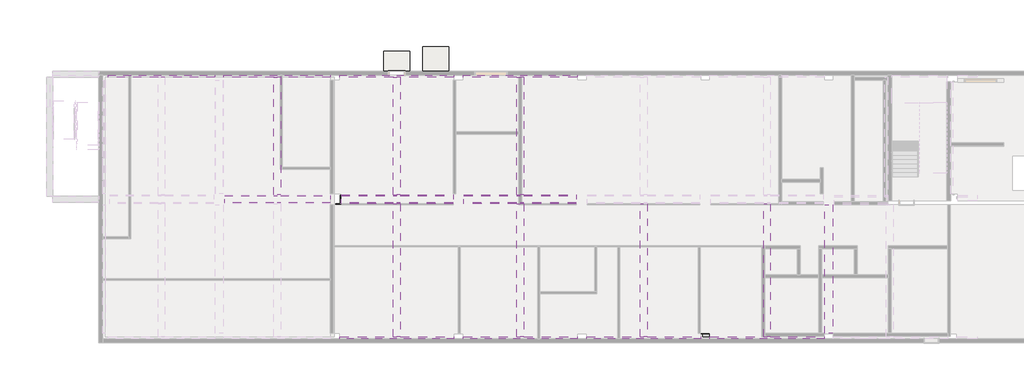
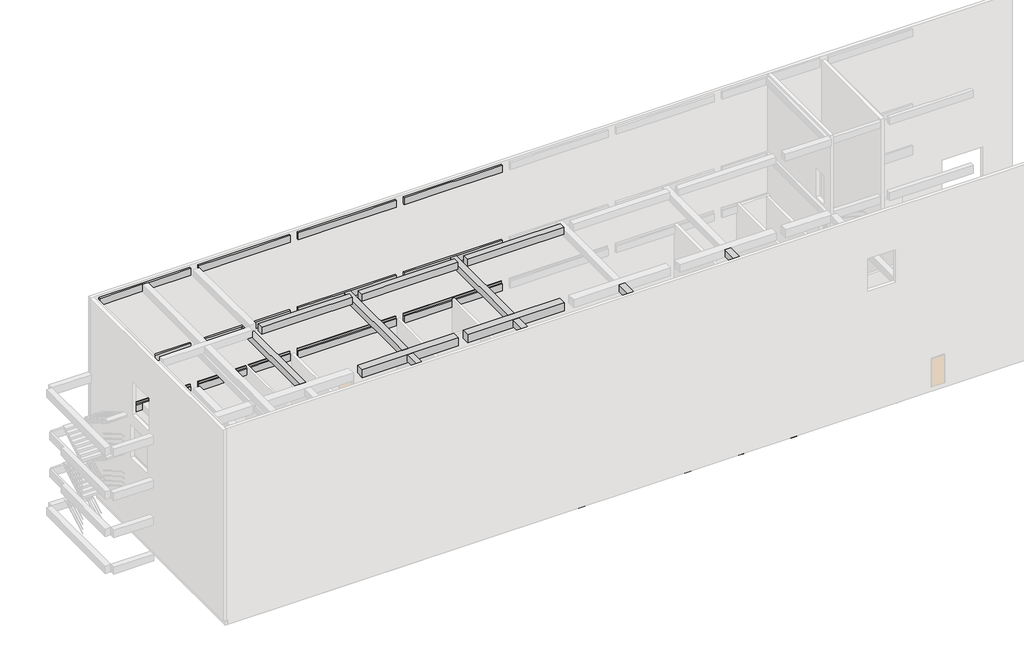
# One storey, part 3 of 5: 54 beams, 2 slabs.
# Revit data of these elements (continued)
# Room at (45344.344, 10064.78) mm, phase "New Construction", upper level "TOC", upper offset 3000 mm, lower offset 0 mm (continued)
#   H_Wall-Base Material-3 = ""
#   H_Floor-Base Material-1 = "Concrete Slab"
#   H_Floor-Base Material-2 = "Steel Trowel Finish"
#   H_Floor-Base Material-3 = ""
#   H_Floor-Base Material-4 = "Concrete Slab"
#   H_Floor-Base Material-5 = ""
#   H_Floor Finish-1 = "Screed"
#   H_Floor Finish-2 = ""
#   H_Floor Finish Remark = "Vinyl Tile"
#   H_Skirt Base Material = "Same as Wall"
#   H_Skirt-Base Material-1 = ""
#   H_Skirt-Base Material-2 = ""
#   H_Skirt-Base Material-3 = ""
#   H_Skirt-Base Material-4 = ""
#   H_Skirt-Base Material-5 = ""
#   H_Skirt Finish-1 = "Vinyl Tile"
#   H_Skirt Finish-2 = ""
#   H_Wall Finish Style Name = "Water Emulsion Paint"
#   H_Wall Base Material = "Masonry Wall / Cement Plaster"
#   H_Wall-Base Material-4 = ""
#   H_Wall-Base Material-5 = ""
#   H_Wall Finish-1 = "Water Emulsion Paint"
#   H_Wall Finish-2 = ""
#   H_Ceiling Finish Style Name = "Suspended Gypsum Plaster Board Ceiling (M-Bar)"
#   H_Ceiling Base Material = "Concrete Slab / Fair Faced Concrete"
#   H_Ceiling-Base Material-1 = "(Concrete Slab)"
#   H_Ceiling-Base Material-2 = "(Fair Faced Concrete)"
#   H_Ceiling-Base Material-3 = ""
#   H_Ceiling-Base Material-4 = ""
#   H_Ceiling-Base Material-5 = "Gypsum Plaster Board Ceiling System"
#   H_Ceiling Finish-1 = "Gypsum Plaster Board Ceiling System"
#   H_Ceiling Finish-2 = ""
#   H_Room W = 4700 mm
#   H_Room L = 8400 mm
#   H_Room H or CH = 3000 mm
#   Floor Finish Style No = F34B
#   Skirt Finish Style No = B35
#   Wall Finish Style No = W02A
#   Ceiling Finish Style No = C92
# Room at (49621.297, 12708.408) mm, phase "New Construction", upper level "TOC", upper offset 2700 mm, lower offset 0 mm
#   Comments = ""
#   Number = "109"
#   Name = "SHOWER ROOM"
#   H_Floor Finish Style Name = "Non-Slip Unglazed Ceramic Tile"
#   H_Floor Base Material = "Concrete Slab / Screed / Liquid Waterproof Membrane"
#   H_Wall-Base Material-1 = "Masonry Wall"
#   H_Skirt Finish Style Name = "Coved Vinyl Tile"
#   H_Wall-Base Material-2 = ""
#   H_Wall-Base Material-3 = ""
#   H_Floor-Base Material-1 = "Concrete Slab"
#   H_Floor-Base Material-2 = ""
#   H_Floor-Base Material-3 = "Screed"
#   H_Floor-Base Material-4 = "Concrete Slab"
#   H_Floor-Base Material-5 = ""
#   H_Floor Finish-1 = "Screed"
#   H_Floor Finish-2 = "Waterproof Membrane"
#   H_Floor Finish Remark = "Ceramic Tile"
#   H_Skirt Base Material = "Same as Wall"
#   H_Skirt-Base Material-1 = ""
#   H_Skirt-Base Material-2 = ""
#   H_Skirt-Base Material-3 = ""
#   H_Skirt-Base Material-4 = ""
#   H_Skirt-Base Material-5 = ""
#   H_Skirt Finish-1 = "Vinyl Tile"
#   H_Skirt Finish-2 = ""
#   H_Wall Finish Style Name = "Glazed Ceramic Tile (≤C.H+100) / No Paint (>C.H+100)"
#   H_Wall Base Material = "Masonry Wall / Waterproof Membrane"
#   H_Wall-Base Material-4 = "Waterproof Membrane"
#   H_Wall-Base Material-5 = "Glazed Ceramic Tile"
#   H_Wall Finish-1 = "Glazed Ceramic Tile"
#   H_Wall Finish-2 = ""
#   H_Ceiling Finish Style Name = "Suspended Acoustic Tiled Ceiling (M-Bar)"
#   H_Ceiling Base Material = "Concrete Slab / Fair Faced Concrete"
#   H_Ceiling-Base Material-1 = "(Concrete Slab)"
#   H_Ceiling-Base Material-2 = "(Fair Faced Concrete)"
#   H_Ceiling-Base Material-3 = ""
#   H_Ceiling-Base Material-4 = ""
#   H_Ceiling-Base Material-5 = "Acoustic Tiled Ceiling System (M-Bar)"
#   H_Ceiling Finish-1 = "Acoustic Tiled Ceiling System (M-Bar)"
#   H_Ceiling Finish-2 = ""
#   H_Room W = 2700 mm
#   H_Room L = 1400 mm
#   H_Room H or CH = 2700 mm
#   Floor Finish Style No = F31C
#   Skirt Finish Style No = none
#   Wall Finish Style No = W32F
#   Ceiling Finish Style No = C95A
# Room at (52871.108, 13591.136) mm, phase "New Construction", upper level "TOC", upper offset 5800 mm, lower offset 0 mm
#   Comments = ""
#   Number = "110"
#   Name = "STAIRCASE"
#   H_Floor Finish Style Name = "Vinyl Tile"
#   H_Floor Base Material = "Concrete Slab / Steel Trowel Finish"
#   H_Wall-Base Material-1 = "Concrete Wall"
#   H_Skirt Finish Style Name = "Coved Vinyl Tile"
#   H_Wall-Base Material-2 = "(Fair Faced Concrete)"
#   H_Wall-Base Material-3 = ""
#   H_Floor-Base Material-1 = "Concrete Slab"
#   H_Floor-Base Material-2 = "Steel Trowel Finish"
#   H_Floor-Base Material-3 = ""
#   H_Floor-Base Material-4 = "Concrete Slab"
#   H_Floor-Base Material-5 = "Steel Trowel Finish"
#   H_Floor Finish-1 = ""
#   H_Floor Finish-2 = ""
#   H_Floor Finish Remark = "Vinyl Tile"
#   H_Skirt Base Material = "Same as Wall"
#   H_Skirt-Base Material-1 = ""
#   H_Skirt-Base Material-2 = ""
#   H_Skirt-Base Material-3 = ""
#   H_Skirt-Base Material-4 = ""
#   H_Skirt-Base Material-5 = ""
#   H_Skirt Finish-1 = "Vinyl Tile"
#   H_Skirt Finish-2 = ""
#   H_Wall Finish Style Name = "Acrylic Emulsion Paint"
#   H_Wall Base Material = "Concrete Wall / Fair Faced Concrete"
#   H_Wall-Base Material-4 = ""
#   H_Wall-Base Material-5 = ""
#   H_Wall Finish-1 = "Acrylic Emulsion Paint"
#   H_Wall Finish-2 = ""
#   H_Ceiling Finish Style Name = "Acrylic Emulsion Paint"
#   H_Ceiling Base Material = "Concrete Slab / Fair Faced Concrete"
#   H_Ceiling-Base Material-1 = "(Concrete Slab)"
#   H_Ceiling-Base Material-2 = ""
#   H_Ceiling-Base Material-3 = ""
#   H_Ceiling-Base Material-4 = ""
#   H_Ceiling-Base Material-5 = ""
#   H_Ceiling Finish-1 = "Acrylic Emulsion Paint"
#   H_Ceiling Finish-2 = ""
#   H_Room W = 2000 mm
#   H_Room L = 8000 mm
#   H_Room H or CH = 5800 mm
#   Floor Finish Style No = F34A
#   Skirt Finish Style No = B35
#   Wall Finish Style No = W01A
#   Ceiling Finish Style No = C01
# Room at (56962.839, 14779.531) mm, phase "New Construction", upper level "TOC", upper offset 5800 mm, lower offset 0 mm
#   Comments = ""
#   Number = "124"
#   Name = "F.O TANK ROOM"
#   H_Floor Finish Style Name = "Non-Slip Epoxy Paint"
#   H_Floor Base Material = "Concrete Slab / Steel Trowel Finish"
#   H_Wall-Base Material-1 = "Concrete Wall"
#   H_Skirt Finish Style Name = "Epoxy Paint"
#   H_Wall-Base Material-2 = "(Fair Faced Concrete)"
#   H_Wall-Base Material-3 = ""
#   H_Floor-Base Material-1 = "Concrete Slab"
#   H_Floor-Base Material-2 = "Steel Trowel Finish"
#   H_Floor-Base Material-3 = ""
#   H_Floor-Base Material-4 = "Concrete Slab"
#   H_Floor-Base Material-5 = "Steel Trowel Finish"
#   H_Floor Finish-1 = ""
#   H_Floor Finish-2 = ""
#   H_Floor Finish Remark = ""
#   H_Skirt Base Material = "Same as Wall"
#   H_Skirt-Base Material-1 = ""
#   H_Skirt-Base Material-2 = ""
#   H_Skirt-Base Material-3 = ""
#   H_Skirt-Base Material-4 = ""
#   H_Skirt-Base Material-5 = ""
#   H_Skirt Finish-1 = "Epoxy Paint"
#   H_Skirt Finish-2 = ""
#   H_Wall Finish Style Name = "Acrylic Emulsion Paint"
#   H_Wall Base Material = "Masonry Wall / Cement Plaster"
#   H_Wall-Base Material-4 = ""
#   H_Wall-Base Material-5 = ""
#   H_Wall Finish-1 = "Acrylic Emulsion Paint"
#   H_Wall Finish-2 = ""
#   H_Ceiling Finish Style Name = "Acrylic Emulsion Paint"
#   H_Ceiling Base Material = "Concrete Slab / Fair Faced Concrete"
#   H_Ceiling-Base Material-1 = "(Concrete Slab)"
#   H_Ceiling-Base Material-2 = ""
#   H_Ceiling-Base Material-3 = ""
#   H_Ceiling-Base Material-4 = ""
#   H_Ceiling-Base Material-5 = ""
#   H_Ceiling Finish-1 = "Acrylic Emulsion Paint"
#   H_Ceiling Finish-2 = ""
#   H_Room W = 3800 mm
#   H_Room L = 8400 mm
#   H_Room H or CH = 5800 mm
#   Floor Finish Style No = F06A
#   Skirt Finish Style No = B03
#   Wall Finish Style No = W01A
#   Ceiling Finish Style No = C01
# Room at (61954.58, 4867.401) mm, phase "New Construction", upper level "TOC", upper offset 5800 mm, lower offset 0 mm
#   Comments = ""
#   Number = "125"
#   Name = "HVAC ROOM"
#   H_Floor Finish Style Name = "Non-Slip Epoxy Paint"
#   H_Floor Base Material = "Concrete Slab / Steel Trowel Finish"
#   H_Wall-Base Material-1 = "Concrete Wall"
#   H_Skirt Finish Style Name = "Epoxy Paint"
#   H_Wall-Base Material-2 = "(Fair Faced Concrete)"
#   H_Wall-Base Material-3 = ""
#   H_Floor-Base Material-1 = "Concrete Slab"
#   H_Floor-Base Material-2 = "Steel Trowel Finish"
#   H_Floor-Base Material-3 = ""
#   H_Floor-Base Material-4 = "Concrete Slab"
#   H_Floor-Base Material-5 = "Steel Trowel Finish"
#   H_Floor Finish-1 = ""
#   H_Floor Finish-2 = ""
#   H_Floor Finish Remark = ""
#   H_Skirt Base Material = "Same as Wall"
#   H_Skirt-Base Material-1 = ""
#   H_Skirt-Base Material-2 = ""
#   H_Skirt-Base Material-3 = ""
#   H_Skirt-Base Material-4 = ""
#   H_Skirt-Base Material-5 = ""
#   H_Skirt Finish-1 = "Epoxy Paint"
#   H_Skirt Finish-2 = ""
#   H_Wall Finish Style Name = "Acrylic Emulsion Paint"
#   H_Wall Base Material = "Masonry Wall / Cement Plaster"
#   H_Wall-Base Material-4 = ""
#   H_Wall-Base Material-5 = ""
#   H_Wall Finish-1 = "Acrylic Emulsion Paint"
#   H_Wall Finish-2 = ""
#   H_Ceiling Finish Style Name = "Suspended Acoustic Tiled Ceiling (M-Bar)"
#   H_Ceiling-Base Material-1 = "(Concrete Slab)"
#   H_Ceiling-Base Material-2 = "(Fair Faced Concrete)"
#   H_Ceiling-Base Material-3 = ""
#   H_Ceiling-Base Material-4 = ""
#   H_Ceiling-Base Material-5 = "Acoustic Tiled Ceiling System (M-Bar)"
#   H_Ceiling Finish-1 = "Acoustic Tiled Ceiling System (M-Bar)"
#   H_Ceiling Finish-2 = ""
#   H_Room W = 3600 mm
#   H_Room L = 4100 mm
#   H_Room H or CH = 5800 mm
#   Floor Finish Style No = F06A
#   Skirt Finish Style No = B03
#   Wall Finish Style No = W01A
#   Ceiling Finish Style No = C95A
# Room at (52877.947, 3986.832) mm, phase "New Construction", upper level "TOC", upper offset 5800 mm, lower offset 0 mm
#   Comments = ""
#   Number = "122"
#   Name = "CYLINDER ROOM (HFC-23)"
#   H_Floor Finish Style Name = "Non-Slip Epoxy Paint"
#   H_Floor Base Material = "Concrete Slab / Steel Trowel Finish"
#   H_Wall-Base Material-1 = "Concrete Wall"
#   H_Skirt Finish Style Name = "Epoxy Paint"
#   H_Wall-Base Material-2 = "(Fair Faced Concrete)"
#   H_Wall-Base Material-3 = ""
#   H_Floor-Base Material-1 = "Concrete Slab"
#   H_Floor-Base Material-2 = "Steel Trowel Finish"
#   H_Floor-Base Material-3 = ""
#   H_Floor-Base Material-4 = "Concrete Slab"
#   H_Floor-Base Material-5 = "Steel Trowel Finish"
#   H_Floor Finish-1 = ""
#   H_Floor Finish-2 = ""
#   H_Floor Finish Remark = ""
#   H_Skirt Base Material = "Same as Wall"
#   H_Skirt-Base Material-1 = ""
#   H_Skirt-Base Material-2 = ""
#   H_Skirt-Base Material-3 = ""
#   H_Skirt-Base Material-4 = ""
#   H_Skirt-Base Material-5 = ""
#   H_Skirt Finish-1 = "Epoxy Paint"
#   H_Skirt Finish-2 = ""
#   H_Wall Finish Style Name = "Acrylic Emulsion Paint"
#   H_Wall Base Material = "Masonry Wall / Cement Plaster"
#   H_Wall-Base Material-4 = ""
#   H_Wall-Base Material-5 = ""
#   H_Wall Finish-1 = "Acrylic Emulsion Paint"
#   H_Wall Finish-2 = ""
#   H_Ceiling Finish Style Name = "Acrylic Emulsion Paint"
#   H_Ceiling Base Material = "Concrete Slab / Fair Faced Concrete"
#   H_Ceiling-Base Material-1 = "(Concrete Slab)"
#   H_Ceiling-Base Material-2 = ""
#   H_Ceiling-Base Material-3 = ""
#   H_Ceiling-Base Material-4 = ""
#   H_Ceiling-Base Material-5 = ""
#   H_Ceiling Finish-1 = "Acrylic Emulsion Paint"
#   H_Ceiling Finish-2 = ""
#   H_Room W = 14300 mm
#   H_Room L = 8900 mm
#   H_Room H or CH = 3000 mm
#   Floor Finish Style No = F06A
#   Skirt Finish Style No = B03
#   Wall Finish Style No = W01A
#   Ceiling Finish Style No = C01
# Room at (47560.665, 5409.289) mm, phase "New Construction", upper level "TOC", upper offset 2700 mm, lower offset 0 mm
#   Comments = ""
#   Number = "119"
#   Name = "DISABLED TOILET(M)"
#   H_Floor Finish Style Name = "Non-Slip Unglazed Ceramic Tile"
#   H_Floor Base Material = "Concrete Slab / Screed / Liquid Waterproofing"
#   H_Wall-Base Material-1 = "Masonry Wall"
#   H_Wall-Base Material-2 = ""
#   H_Wall-Base Material-3 = ""
#   H_Floor-Base Material-1 = "Concrete Slab"
#   H_Floor-Base Material-2 = ""
#   H_Floor-Base Material-3 = "Screed"
#   H_Floor-Base Material-4 = "Concrete Slab"
#   H_Floor-Base Material-5 = ""
#   H_Floor Finish-1 = "Screed"
#   H_Floor Finish-2 = "Liquid Waterproofing"
#   H_Floor Finish Remark = "Ceramic Tile"
#   H_Wall Finish Style Name = "Glazed Ceramic Tile"
#   H_Wall Base Material = "Masonry Wall"
#   H_Wall-Base Material-4 = "Liquid Waterproofing"
#   H_Wall-Base Material-5 = "Glazed Ceramic Tile"
#   H_Wall Finish-1 = "Glazed Ceramic Tile"
#   H_Wall Finish-2 = ""
#   H_Ceiling Finish Style Name = "Suspended Moisture Resistant Tiled Ceiling (M-Bar)"
#   H_Ceiling Base Material = "Concrete Slab / Fair Faced Concrete"
#   H_Ceiling-Base Material-1 = "(Concrete Slab)"
#   H_Ceiling-Base Material-2 = "(Fair Faced Concrete)"
#   H_Ceiling-Base Material-3 = ""
#   H_Ceiling-Base Material-4 = ""
#   H_Ceiling-Base Material-5 = "Moisture Resistant Tiled Ceiling System (M-Bar)"
#   H_Ceiling Finish-1 = "Moisture Resistant Tiled Ceiling System (M-Bar)"
#   H_Ceiling Finish-2 = ""
#   H_Room W = 4400 mm
#   H_Room L = 3700 mm
#   H_Room H or CH = 2700 mm
#   Floor Finish Style No = F31B
#   Wall Finish Style No = W34B
#   Ceiling Finish Style No = C96A
# Room at (44106.126, 5206.081) mm, phase "New Construction", upper level "TOC", upper offset 2700 mm, lower offset 0 mm
#   Comments = ""
#   Number = "118"
#   Name = "DISABLED TOILET(W)"
#   H_Floor Finish Style Name = "Non-Slip Unglazed Ceramic Tile"
#   H_Floor Base Material = "Concrete Slab / Screed / Liquid Waterproofing"
#   H_Wall-Base Material-1 = "Masonry Wall"
#   H_Wall-Base Material-2 = ""
#   H_Wall-Base Material-3 = ""
#   H_Floor-Base Material-1 = "Concrete Slab"
#   H_Floor-Base Material-2 = ""
#   H_Floor-Base Material-3 = "Screed"
#   H_Floor-Base Material-4 = "Concrete Slab"
#   H_Floor-Base Material-5 = ""
#   H_Floor Finish-1 = "Screed"
#   H_Floor Finish-2 = "Liquid Waterproofing"
#   H_Floor Finish Remark = "Ceramic Tile"
#   H_Wall Finish Style Name = "Glazed Ceramic Tile"
#   H_Wall Base Material = "Masonry Wall"
#   H_Wall-Base Material-4 = "Liquid Waterproofing"
#   H_Wall-Base Material-5 = "Glazed Ceramic Tile"
#   H_Wall Finish-1 = "Glazed Ceramic Tile"
#   H_Wall Finish-2 = ""
#   H_Ceiling Finish Style Name = "Suspended Moisture Resistant Tiled Ceiling (M-Bar)"
#   H_Ceiling Base Material = "Concrete Slab / Fair Faced Concrete"
#   H_Ceiling-Base Material-1 = "(Concrete Slab)"
#   H_Ceiling-Base Material-2 = "(Fair Faced Concrete)"
#   H_Ceiling-Base Material-3 = ""
#   H_Ceiling-Base Material-4 = ""
#   H_Ceiling-Base Material-5 = "Moisture Resistant Tiled Ceiling System (M-Bar)"
#   H_Ceiling Finish-1 = "Moisture Resistant Tiled Ceiling System (M-Bar)"
#   H_Ceiling Finish-2 = ""
#   H_Room W = 2300 mm
#   H_Room L = 1900 mm
#   H_Room H or CH = 2700 mm
#   Floor Finish Style No = F31B
#   Wall Finish Style No = W34B
#   Ceiling Finish Style No = C96A
# Room at (44139.994, 3106.263) mm, phase "New Construction", upper level "TOC", upper offset 2700 mm, lower offset 0 mm
#   Comments = ""
#   Number = "120"
#   Name = "TOILET (W)"
#   H_Floor Finish Style Name = "Non-Slip Unglazed Ceramic Tile"
#   H_Floor Base Material = "Concrete Slab / Screed / Liquid Waterproofing"
#   H_Wall-Base Material-1 = "Masonry Wall"
#   H_Wall-Base Material-2 = ""
#   H_Wall-Base Material-3 = ""
#   H_Floor-Base Material-1 = "Concrete Slab"
#   H_Floor-Base Material-2 = ""
#   H_Floor-Base Material-3 = "Screed"
#   H_Floor-Base Material-4 = "Concrete Slab"
#   H_Floor-Base Material-5 = ""
#   H_Floor Finish-1 = "Screed"
#   H_Floor Finish-2 = "Liquid Waterproofing"
#   H_Floor Finish Remark = "Ceramic Tile"
#   H_Wall Finish Style Name = "Glazed Ceramic Tile"
#   H_Wall Base Material = "Masonry Wall"
#   H_Wall-Base Material-4 = "Liquid Waterproofing"
#   H_Wall-Base Material-5 = "Glazed Ceramic Tile"
#   H_Wall Finish-1 = "Glazed Ceramic Tile"
#   H_Wall Finish-2 = ""
#   H_Ceiling Finish Style Name = "Suspended Moisture Resistant Tiled Ceiling (M-Bar)"
#   H_Ceiling Base Material = "Concrete Slab / Fair Faced Concrete"
#   H_Ceiling-Base Material-1 = "(Concrete Slab)"
#   H_Ceiling-Base Material-2 = "(Fair Faced Concrete)"
#   H_Ceiling-Base Material-3 = ""
#   H_Ceiling-Base Material-4 = ""
#   H_Ceiling-Base Material-5 = "Moisture Resistant Tiled Ceiling System (M-Bar)"
#   H_Ceiling Finish-1 = "Moisture Resistant Tiled Ceiling System (M-Bar)"
#   H_Ceiling Finish-2 = ""
#   H_Room W = 2300 mm
#   H_Room L = 1900 mm
#   H_Room H or CH = 2700 mm
#   Floor Finish Style No = F31B
#   Wall Finish Style No = W34B
#   Ceiling Finish Style No = C96A
# Room at (36248.742, 3377.207) mm, phase "New Construction", upper level "TOC", upper offset 3000 mm, lower offset 0 mm
#   Comments = ""
#   Number = "116"
#   Name = "PRESIDENT ROOM"
#   H_Floor Finish Style Name = "Carpet Tile"
#   H_Floor Base Material = "Concrete Slab / Steel Trowel Finish"
#   H_Wall-Base Material-1 = "Concrete Wall"
#   H_Skirt Finish Style Name = "Coved Vinyl Tile"
#   H_Wall-Base Material-2 = "(Fair Faced Concrete)"
#   H_Wall-Base Material-3 = ""
#   H_Floor-Base Material-1 = "Recess Floor Mat"
#   H_Floor-Base Material-2 = ""
#   H_Floor-Base Material-3 = ""
#   H_Floor-Base Material-4 = "Concrete Slab"
#   H_Floor-Base Material-5 = "Steel Trowel Finish"
#   H_Floor Finish-1 = ""
#   H_Floor Finish-2 = ""
#   H_Floor Finish Remark = "Carpet Tile"
#   H_Skirt Base Material = "Same as Wall"
#   H_Skirt-Base Material-1 = ""
#   H_Skirt-Base Material-2 = ""
#   H_Skirt-Base Material-3 = ""
#   H_Skirt-Base Material-4 = ""
#   H_Skirt-Base Material-5 = ""
#   H_Skirt Finish-1 = "Vinyl Tile"
#   H_Skirt Finish-2 = ""
#   H_Wall Finish Style Name = "Water Emulsion Paint"
#   H_Wall Base Material = "Masonry Wall / Cement Plaster"
#   H_Wall-Base Material-4 = ""
#   H_Wall-Base Material-5 = ""
#   H_Wall Finish-1 = "Water Emulsion Paint"
#   H_Wall Finish-2 = ""
#   H_Ceiling Finish Style Name = "Suspended Acoustic Tiled Ceiling (M-Bar)"
#   H_Ceiling Base Material = "Concrete Slab / Fair Faced Concrete"
#   H_Ceiling-Base Material-1 = "(Concrete Slab)"
#   H_Ceiling-Base Material-2 = "(Fair Faced Concrete)"
#   H_Ceiling-Base Material-3 = ""
#   H_Ceiling-Base Material-4 = ""
#   H_Ceiling-Base Material-5 = "Acoustic Tiled Ceiling System (M-Bar)"
#   H_Ceiling Finish-1 = "Acoustic Tiled Ceiling System (M-Bar)"
#   H_Ceiling Finish-2 = ""
#   H_Room W = 8000 mm
#   H_Room L = 6100 mm
#   H_Room H or CH = 3000 mm
#   Floor Finish Style No = F43
#   Skirt Finish Style No = B35
#   Wall Finish Style No = W02A
#   Ceiling Finish Style No = C95A
# Room at (30050.892, 2259.562) mm, phase "New Construction", upper level "TOC", upper offset 3000 mm, lower offset 0 mm
#   Comments = ""
#   Number = "114"
#   Name = "STORAGE"
#   H_Floor Finish Style Name = "Vinyl Tile"
#   H_Floor Base Material = "Concrete Slab / Steel Trowel Finish"
#   H_Wall-Base Material-1 = "Masonry Wall"
#   H_Skirt Finish Style Name = "Coved Vinyl Tile"
#   H_Wall-Base Material-2 = ""
#   H_Wall-Base Material-3 = "Plastering"
#   H_Floor-Base Material-1 = "Concrete Slab"
#   H_Floor-Base Material-2 = "Steel Trowel Finish"
#   H_Floor-Base Material-3 = ""
#   H_Floor-Base Material-4 = "Concrete Slab"
#   H_Floor-Base Material-5 = "Steel Trowel Finish"
#   H_Floor Finish-1 = ""
#   H_Floor Finish-2 = ""
#   H_Floor Finish Remark = "Vinyl Tile"
#   H_Skirt Base Material = "Same as Wall"
#   H_Skirt-Base Material-1 = ""
#   H_Skirt-Base Material-2 = ""
#   H_Skirt-Base Material-3 = ""
#   H_Skirt-Base Material-4 = ""
#   H_Skirt-Base Material-5 = ""
#   H_Skirt Finish-1 = "Vinyl Tile"
#   H_Skirt Finish-2 = ""
#   H_Skirt Finish Remark = "Vinyl Tile = PVC Tile (polyvinyl chloride)"
#   H_Wall Finish Style Name = "Water Emulsion Paint"
#   H_Wall Base Material = "Masonry Wall / Cement Plaster"
#   H_Wall-Base Material-4 = ""
#   H_Wall-Base Material-5 = ""
#   H_Wall Finish-1 = ""
#   H_Wall Finish-2 = ""
#   H_Wall Finish Remark = ""
#   H_Ceiling Finish Style Name = "Suspended Gypsum Plaster Board Ceiling (M-Bar)"
#   H_Ceiling Base Material = "Concrete Slab / Fair Faced Concrete"
#   H_Ceiling-Base Material-1 = "(Concrete Slab)"
#   H_Ceiling-Base Material-2 = "(Fair Faced Concrete)"
#   H_Ceiling-Base Material-3 = ""
#   H_Ceiling-Base Material-4 = ""
#   H_Ceiling-Base Material-5 = "Gypsum Plaster Board Ceiling System"
#   H_Ceiling Finish-1 = "Gypsum Plaster Board Ceiling System"
#   H_Ceiling Finish-2 = ""
#   H_Room W = 5200 mm
#   H_Room L = 6100 mm
#   H_Room H or CH = 3000 mm
#   Floor Finish Style No = F34A
#   Skirt Finish Style No = none
#   Wall Finish Style No = none
#   Ceiling Finish Style No = C92
# Room at (30017.024, 4901.269) mm, phase "New Construction", upper level "TOC", upper offset 3000 mm, lower offset 0 mm
#   Comments = ""
#   Number = "113"
#   Name = "MAAMS REST ROOM"
#   H_Floor Finish Style Name = "Vinyl Tile"
#   H_Floor Base Material = "Concrete Slab / Screed"
#   H_Wall-Base Material-1 = "Concrete Wall"
#   H_Skirt Finish Style Name = "Coved Vinyl Tile"
#   H_Wall-Base Material-2 = "(Fair Faced Concrete)"
#   H_Wall-Base Material-3 = ""
#   H_Floor-Base Material-1 = "Concrete Slab"
#   H_Floor-Base Material-2 = "Steel Trowel Finish"
#   H_Floor-Base Material-3 = ""
#   H_Floor-Base Material-4 = "Concrete Slab"
#   H_Floor-Base Material-5 = ""
#   H_Floor Finish-1 = "Screed"
#   H_Floor Finish-2 = ""
#   H_Floor Finish Remark = "Vinyl Tile"
#   H_Skirt Base Material = "Same as Wall"
#   H_Skirt-Base Material-1 = ""
#   H_Skirt-Base Material-2 = ""
#   H_Skirt-Base Material-3 = ""
#   H_Skirt-Base Material-4 = ""
#   H_Skirt-Base Material-5 = ""
#   H_Skirt Finish-1 = "Vinyl Tile"
#   H_Skirt Finish-2 = ""
#   H_Wall Finish Style Name = "Water Emulsion Paint"
#   H_Wall Base Material = "Masonry Wall / Cement Plaster"
#   H_Wall-Base Material-4 = ""
#   H_Wall-Base Material-5 = ""
#   H_Wall Finish-1 = "Water Emulsion Paint"
#   H_Wall Finish-2 = ""
#   H_Ceiling Finish Style Name = "Suspended Gypsum Plaster Board Ceiling (M-Bar)"
#   H_Ceiling Base Material = "Concrete Slab / Fair Faced Concrete"
#   H_Ceiling-Base Material-1 = "(Concrete Slab)"
#   H_Ceiling-Base Material-2 = "(Fair Faced Concrete)"
#   H_Ceiling-Base Material-3 = ""
#   H_Ceiling-Base Material-4 = ""
#   H_Ceiling-Base Material-5 = "Gypsum Plaster Board Ceiling System"
#   H_Ceiling Finish-1 = "Gypsum Plaster Board Ceiling System"
#   H_Ceiling Finish-2 = ""
#   H_Room W = 5200 mm
#   H_Room L = 6100 mm
#   H_Room H or CH = 3000 mm
#   Floor Finish Style No = F34B
#   Skirt Finish Style No = B35
#   Wall Finish Style No = W02A
#   Ceiling Finish Style No = C92
# Room at (19246.99, 3580.415) mm, phase "New Construction", upper level "TOC", upper offset 3000 mm, lower offset 0 mm
#   Comments = ""
#   Number = "112"
#   Name = "CONFERENCE ROOM"
#   H_Floor Finish Style Name = "Carpet Tile"
#   H_Floor Base Material = "Concrete Slab / Steel Trowel Finish"
#   H_Wall-Base Material-1 = "Concrete Wall"
#   H_Skirt Finish Style Name = "Coved Vinyl Tile"
#   H_Wall-Base Material-2 = "(Fair Faced Concrete)"
#   H_Wall-Base Material-3 = ""
#   H_Floor-Base Material-1 = "Recess Floor Mat"
#   H_Floor-Base Material-2 = ""
#   H_Floor-Base Material-3 = ""
#   H_Floor-Base Material-4 = "Concrete Slab"
#   H_Floor-Base Material-5 = "Steel Trowel Finish"
#   H_Floor Finish-1 = ""
#   H_Floor Finish-2 = ""
#   H_Floor Finish Remark = "Carpet Tile"
#   H_Skirt Base Material = "Same as Wall"
#   H_Skirt-Base Material-1 = ""
#   H_Skirt-Base Material-2 = ""
#   H_Skirt-Base Material-3 = ""
#   H_Skirt-Base Material-4 = ""
#   H_Skirt-Base Material-5 = ""
#   H_Skirt Finish-1 = "Vinyl Tile"
#   H_Skirt Finish-2 = ""
#   H_Wall Finish Style Name = "Water Emulsion Paint"
#   H_Wall Base Material = "Masonry Wall / Cement Plaster"
#   H_Wall-Base Material-4 = ""
#   H_Wall-Base Material-5 = ""
#   H_Wall Finish-1 = "Water Emulsion Paint"
#   H_Wall Finish-2 = ""
#   H_Ceiling Finish Style Name = "Suspended Acoustic Tiled Ceiling (M-Bar)"
#   H_Ceiling Base Material = "Concrete Slab / Fair Faced Concrete"
#   H_Ceiling-Base Material-1 = "(Concrete Slab)"
#   H_Ceiling-Base Material-2 = "(Fair Faced Concrete)"
#   H_Ceiling-Base Material-3 = ""
#   H_Ceiling-Base Material-4 = ""
#   H_Ceiling-Base Material-5 = "Acoustic Tiled Ceiling System (M-Bar)"
#   H_Ceiling Finish-1 = "Acoustic Tiled Ceiling System (M-Bar)"
#   H_Ceiling Finish-2 = ""
#   H_Room W = 5100 mm
#   H_Room L = 6100 mm
#   H_Room H or CH = 3000 mm
#   Floor Finish Style No = F43
#   Skirt Finish Style No = B35
#   Wall Finish Style No = W02A
#   Ceiling Finish Style No = C95A
# Room at (61369.572, 13806.461) mm, phase "New Construction", upper level "TOC", upper offset 9300 mm, lower offset 0 mm
#   Comments = ""
#   Number = "123"
#   Name = "EDG ROOM"
#   H_Floor Finish Style Name = "Non-Slip Epoxy Paint"
#   H_Floor Base Material = "Concrete Slab / Steel Trowel Finish"
#   H_Wall-Base Material-1 = "Concrete Wall"
#   H_Skirt Finish Style Name = "Epoxy Paint"
#   H_Wall-Base Material-2 = "(Fair Faced Concrete)"
#   H_Wall-Base Material-3 = ""
#   H_Floor-Base Material-1 = "Concrete Slab"
#   H_Floor-Base Material-2 = "Steel Trowel Finish"
#   H_Floor-Base Material-3 = ""
#   H_Floor-Base Material-4 = "Concrete Slab"
#   H_Floor-Base Material-5 = "Steel Trowel Finish"
#   H_Floor Finish-1 = ""
#   H_Floor Finish-2 = ""
#   H_Floor Finish Remark = ""
#   H_Skirt Base Material = "Same as Wall"
#   H_Skirt-Base Material-1 = ""
#   H_Skirt-Base Material-2 = ""
#   H_Skirt-Base Material-3 = ""
#   H_Skirt-Base Material-4 = ""
#   H_Skirt-Base Material-5 = ""
#   H_Skirt Finish-1 = "Epoxy Paint"
#   H_Skirt Finish-2 = ""
#   H_Wall Finish Style Name = "Acrylic Emulsion Paint"
#   H_Wall Base Material = "Masonry Wall / Cement Plaster"
#   H_Wall-Base Material-4 = ""
#   H_Wall-Base Material-5 = ""
#   H_Wall Finish-1 = "Acrylic Emulsion Paint"
#   H_Wall Finish-2 = ""
#   H_Ceiling Finish Style Name = "Acrylic Emulsion Paint"
#   H_Ceiling Base Material = "Concrete Slab / Fair Faced Concrete"
#   H_Ceiling-Base Material-1 = "(Concrete Slab)"
#   H_Ceiling-Base Material-2 = ""
#   H_Ceiling-Base Material-3 = ""
#   H_Ceiling-Base Material-4 = ""
#   H_Ceiling-Base Material-5 = ""
#   H_Ceiling Finish-1 = "Acrylic Emulsion Paint"
#   H_Ceiling Finish-2 = ""
#   H_Room W = 8200 mm
#   H_Room L = 6100 mm
#   H_Room H or CH = 9300 mm
#   Floor Finish Style No = F06A
#   Skirt Finish Style No = B03
#   Wall Finish Style No = W01A
#   Ceiling Finish Style No = C01
# Room at (33987.4, 7910.137) mm, phase "New Construction", upper level "TOC", upper offset 3000 mm, lower offset 0 mm
#   Comments = ""
#   Number = "111"
#   Name = "CORRIDOR"
#   H_Floor Finish Style Name = "Vinyl Tile"
#   H_Floor Base Material = "Concrete Slab / Steel Trowel Finish"
#   H_Wall-Base Material-1 = "Concrete Wall"
#   H_Skirt Finish Style Name = "Coved Vinyl Tile"
#   H_Wall-Base Material-2 = "(Fair Faced Concrete)"
#   H_Wall-Base Material-3 = ""
#   H_Floor-Base Material-1 = "Concrete Slab"
#   H_Floor-Base Material-2 = "Steel Trowel Finish"
#   H_Floor-Base Material-3 = ""
#   H_Floor-Base Material-4 = "Concrete Slab"
#   H_Floor-Base Material-5 = "Steel Trowel Finish"
#   H_Floor Finish-1 = ""
#   H_Floor Finish-2 = ""
#   H_Floor Finish Remark = "Vinyl Tile"
#   H_Skirt Base Material = "Same as Wall"
#   H_Skirt-Base Material-1 = ""
#   H_Skirt-Base Material-2 = ""
#   H_Skirt-Base Material-3 = ""
#   H_Skirt-Base Material-4 = ""
#   H_Skirt-Base Material-5 = ""
#   H_Skirt Finish-1 = "Vinyl Tile"
#   H_Skirt Finish-2 = ""
#   H_Wall Finish Style Name = "Water Emulsion Paint"
#   H_Wall Base Material = "Masonry Wall / Cement Plaster"
#   H_Wall-Base Material-4 = ""
#   H_Wall-Base Material-5 = ""
#   H_Wall Finish-1 = "Water Emulsion Paint"
#   H_Wall Finish-2 = ""
#   H_Ceiling Finish Style Name = "Suspended Gypsum Plaster Board Ceiling (M-Bar)"
#   H_Ceiling Base Material = "Concrete Slab / Fair Faced Concrete"
#   H_Ceiling-Base Material-1 = "(Concrete Slab)"
#   H_Ceiling-Base Material-2 = "(Fair Faced Concrete)"
#   H_Ceiling-Base Material-3 = ""
#   H_Ceiling-Base Material-4 = ""
#   H_Ceiling-Base Material-5 = "Gypsum Plaster Board Ceiling System"
#   H_Ceiling Finish-1 = "Gypsum Plaster Board Ceiling System"
#   H_Ceiling Finish-2 = ""
#   H_Room W = 14400 mm
#   H_Room L = 8400 mm
#   H_Room H or CH = 3000 mm
#   Floor Finish Style No = F34A
#   Skirt Finish Style No = B35
#   Wall Finish Style No = W02A
#   Ceiling Finish Style No = C92
